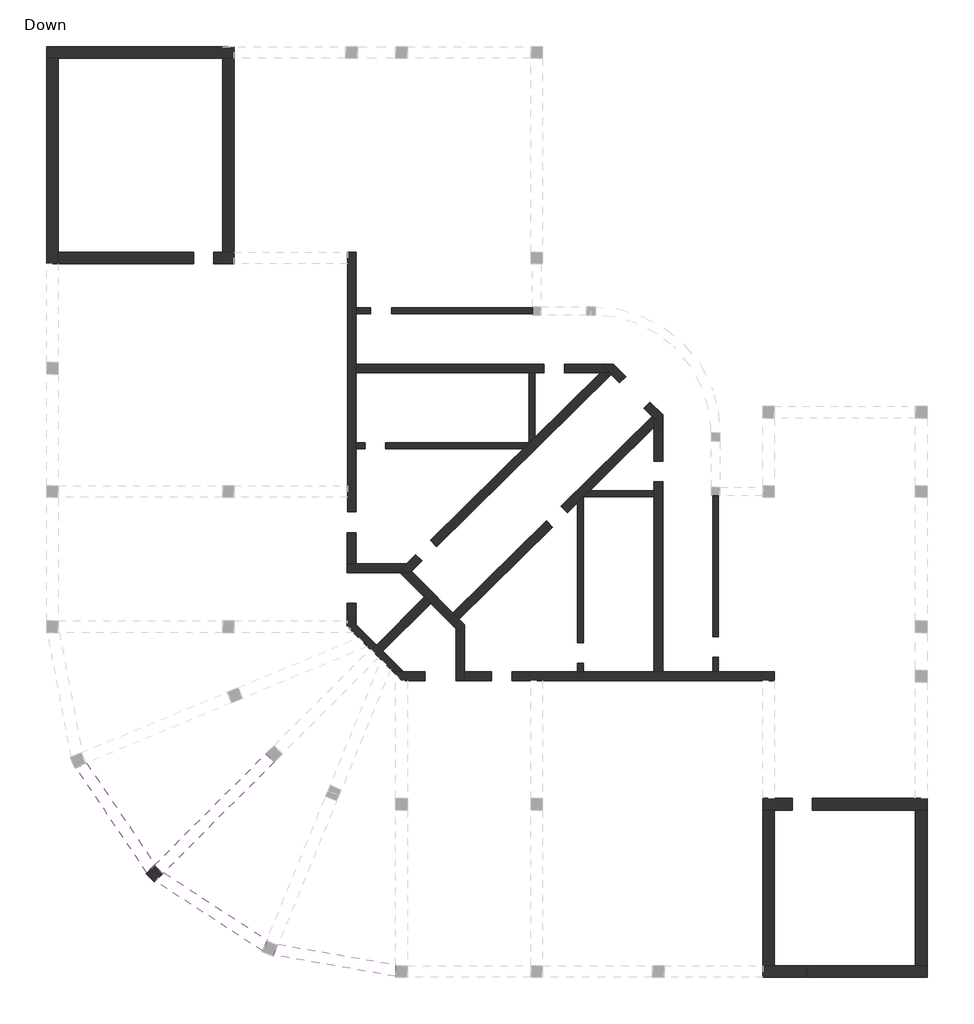
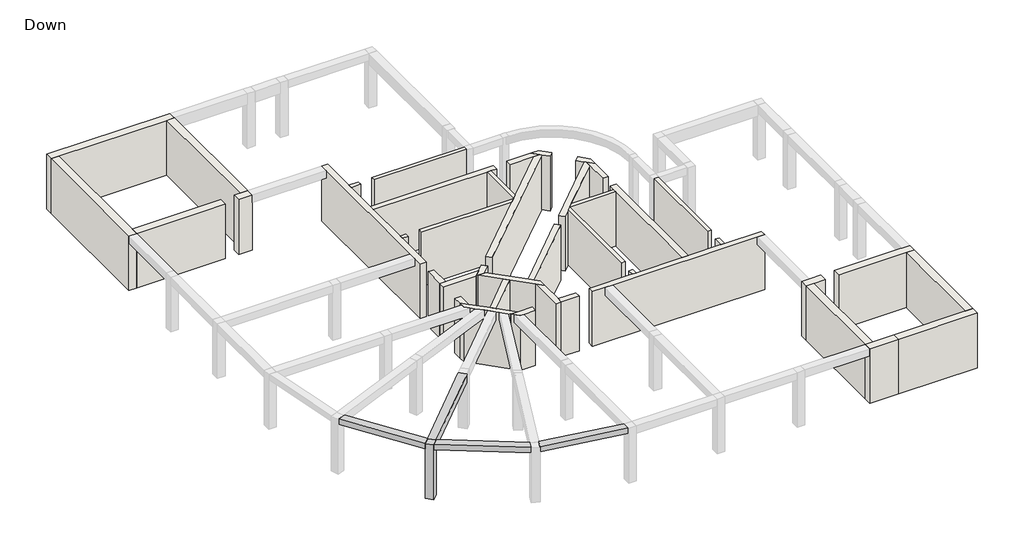
# One storey, part 1 of 2: 42 walls, 4 beams, 1 column.
"""IFC4 building model written with IfcOpenShell, lengths in millimetres."""

from ifc_helpers import new_model, si_unit, origin, origin_with_axes, place, context, project, spatial, polyline, outline, extrude, faceted_brep, element, save

model = new_model("IFC4")

# Units and contexts
model_context = context("Model", 3, world=origin())
ifc_project = project(units=[si_unit("LENGTHUNIT", "METRE", prefix="MILLI")], contexts=[model_context])

# Site, building, storey
site = spatial("IfcSite", under=ifc_project)
building = spatial("IfcBuilding", under=site)
storey = spatial("IfcBuildingStorey", under=building, Name="Down", Elevation=0.0)

# Beams
placement = place(None, origin())
element("IfcBeam", 1, ObjectType="Concrete Rectengular Beam : 39/30", at=placement, inside=storey, context=model_context, shape_type="Brep", body=[
    faceted_brep([(-10715.118829, -3249.9785454, 3000.0), (-10744.371321, -3279.2310368, 3000.0), (-10997.081006, -3531.9407164, 3000.0), (-7342.0637038, -5902.9717923, 3000.0), (-7204.9594265, -5567.8069151, 3000.0), (-7191.7801663, -5535.5889186, 3000.0), (-7191.7801663, -5535.5889186, 2800.0), (-7191.7801663, -5535.5889186, 2700.0), (-10715.118829, -3249.9785454, 2700.0), (-10715.118829, -3249.9785454, 2800.0), (-10997.081006, -3531.9407164, 2700.0), (-7342.0637038, -5902.9717923, 2700.0)], [[[0, 1, 2, 3, 4, 5]], [[0, 5, 6, 7, 8, 9]], [[10, 8, 7, 11]], [[2, 10, 11, 3]], [[10, 2, 1, 0, 9, 8]], [[3, 11, 7, 6, 5, 4]]]),
])
element("IfcBeam", 2, ObjectType="Concrete Rectengular Beam : 39/30", at=placement, inside=storey, context=model_context, shape_type="Brep", body=[
    faceted_brep([(-13331.7826338, 480.4747094, 3000.0), (-13367.6133817, 465.6307069, 3000.0), (-13699.4952625, 328.1383075, 3000.0), (-11282.6282398, -3251.8025252, 3000.0), (-11027.2140258, -2996.3883167, 3000.0), (-11001.7177394, -2970.8920309, 3000.0), (-11001.7177394, -2970.8920309, 2800.0), (-11001.7177394, -2970.8920309, 2700.0), (-13331.7826338, 480.4747094, 2700.0), (-13331.7826338, 480.4747094, 2800.0), (-13699.4952625, 328.1383075, 2700.0), (-11282.6282398, -3251.8025252, 2700.0)], [[[0, 1, 2, 3, 4, 5]], [[0, 5, 6, 7, 8, 9]], [[10, 8, 7, 11]], [[2, 10, 11, 3]], [[10, 2, 1, 0, 9, 8]], [[3, 11, 7, 6, 5, 4]]]),
])
element("IfcBeam", 3, ObjectType="Concrete Rectengular Beam : 39/30", at=placement, inside=storey, context=model_context, shape_type="Brep", body=[
    faceted_brep([(-2813.8658054, -6775.1305116, 3000.0), (-2813.8658054, -6410.076772, 3000.0), (-2813.8658054, -6379.2217224, 3000.0), (-6818.4727302, -5679.49154, 3000.0), (-6834.7373046, -5719.2518901, 3000.0), (-6969.6216332, -6048.9898845, 3000.0), (-2813.8658054, -6775.1305116, 2700.0), (-6969.6216332, -6048.9898845, 2700.0), (-2813.8658054, -6379.2217224, 2700.0), (-6818.4727302, -5679.49154, 2700.0), (-2813.8658054, -6379.2217224, 2800.0), (-6818.4727302, -5679.49154, 2800.0)], [[[0, 1, 2, 3, 4, 5]], [[6, 0, 5, 7]], [[8, 6, 7, 9]], [[3, 2, 10, 8, 9, 11]], [[0, 6, 8, 10, 2, 1]], [[7, 5, 4, 3, 11, 9]]]),
])
element("IfcBeam", 4, ObjectType="Concrete Rectengular Beam : 40/40", at=placement, inside=storey, context=model_context, shape_type="Brep", body=[
    faceted_brep([(-11027.2140255, -2996.388317, 3000.0), (-10744.3713207, -3279.2310371, 3000.0), (-10715.118829, -3249.9785454, 3000.0), (-6954.333921, 510.8063626, 3000.0), (-7237.1766258, 793.6490827, 3000.0), (-11001.7177394, -2970.8920309, 3000.0), (-10744.3713207, -3279.2310371, 2600.0), (-6954.333921, 510.8063626, 2600.0), (-6954.333921, 510.8063626, 2800.0), (-11027.2140255, -2996.388317, 2600.0), (-7237.1766258, 793.6490827, 2600.0), (-7237.1766258, 793.6490827, 2800.0)], [[[0, 1, 2, 3, 4, 5]], [[1, 6, 7, 8, 3, 2]], [[6, 9, 10, 7]], [[9, 0, 5, 4, 11, 10]], [[1, 0, 9, 6]], [[4, 3, 8, 7, 10, 11]]]),
])

# Column
element("IfcColumn", 5, ObjectType="Concrete Rectengular Column : 40/40", at=placement, inside=storey, context=model_context, shape_type="SweptSolid", body=[
    extrude(outline(polyline([(-10744.3713169, -3279.2310409), (-11027.2140369, -3562.0737458), (-11310.0567418, -3279.2310257), (-11027.2140217, -2996.3883208), (-10744.3713169, -3279.2310409)])), origin_with_axes(), (0.0, 0.0, 1.0), 3000.0),
])

# Walls
element("IfcWall", 6, ObjectType="20", at=placement, inside=storey, context=model_context, shape_type="Brep", body=[
    faceted_brep([(-4161.7067397, 15761.3377606, 0.0), (-3665.2660617, 15761.3377606, 0.0), (-3665.2660617, 15761.3377606, 2800.0), (-3665.2660617, 15761.3377606, 3000.0), (-4161.7067397, 15761.3377606, 3000.0), (-4161.7067397, 15761.3377606, 2800.0), (-4161.7067397, 15961.3377606, 0.0), (-4161.7067397, 15961.3377606, 2800.0), (-4161.7067397, 15961.3377606, 3000.0), (-3665.2660617, 15961.3377606, 3000.0), (-3665.2660617, 15961.3377606, 2800.0), (-3665.2660617, 15961.3377606, 0.0)], [[[0, 1, 2, 3, 4, 5]], [[6, 7, 8, 9, 10, 11]], [[1, 0, 6, 11]], [[3, 2, 1, 11, 10, 9]], [[4, 3, 9, 8]], [[0, 5, 4, 8, 7, 6]]]),
])
element("IfcWall", 7, ObjectType="20", at=placement, inside=storey, context=model_context, shape_type="Brep", body=[
    faceted_brep([(-2964.398431, 15761.3377606, 0.0), (1829.020722, 15761.3377606, 0.0), (1829.020722, 15761.3377606, 2800.0), (1829.020722, 15761.3377606, 3000.0), (-2964.398431, 15761.3377606, 3000.0), (-2964.398431, 15761.3377606, 2800.0), (-2964.398431, 15961.3377606, 0.0), (-2964.398431, 15961.3377606, 2800.0), (-2964.398431, 15961.3377606, 3000.0), (1829.020722, 15961.3377606, 3000.0), (1829.020722, 15961.3377606, 2800.0), (1829.020722, 15961.3377606, 0.0)], [[[0, 1, 2, 3, 4, 5]], [[6, 7, 8, 9, 10, 11]], [[1, 0, 6, 11]], [[3, 2, 1, 11, 10, 9]], [[4, 3, 9, 8]], [[0, 5, 4, 8, 7, 6]]]),
])
element("IfcWall", 8, ObjectType="20", at=placement, inside=storey, context=model_context, shape_type="Brep", body=[
    faceted_brep([(8168.0773416, 3579.3391577, 0.0), (8168.0773416, 4078.4432768, 0.0), (8168.0773416, 4078.4432768, 2800.0), (8168.0773416, 4078.4432768, 3000.0), (8168.0773416, 3579.3391577, 3000.0), (8168.0773416, 3579.3391577, 2800.0), (7968.0773416, 3579.3391577, 0.0), (7968.0773416, 3579.3391577, 2800.0), (7968.0773416, 3579.3391577, 3000.0), (7968.0773416, 4078.4432768, 3000.0), (7968.0773416, 4078.4432768, 2800.0), (7968.0773416, 4078.4432768, 0.0)], [[[0, 1, 2, 3, 4, 5]], [[6, 7, 8, 9, 10, 11]], [[1, 0, 6, 11]], [[3, 2, 1, 11, 10, 9]], [[4, 3, 9, 8]], [[0, 5, 4, 8, 7, 6]]]),
])
element("IfcWall", 9, ObjectType="20", at=placement, inside=storey, context=model_context, shape_type="Brep", body=[
    faceted_brep([(8168.0773416, 4779.3109075, 0.0), (8168.0773416, 9562.1590026, 0.0), (8168.0773416, 9562.1590026, 2800.0), (8168.0773416, 9562.1590026, 3000.0), (8168.0773416, 4779.3109075, 3000.0), (8168.0773416, 4779.3109075, 2800.0), (7968.0773416, 4779.3109075, 0.0), (7968.0773416, 4779.3109075, 2800.0), (7968.0773416, 4779.3109075, 3000.0), (7968.0773416, 9562.1590026, 3000.0), (7968.0773416, 9562.1590026, 2800.0), (7968.0773416, 9562.1590026, 0.0)], [[[0, 1, 2, 3, 4, 5]], [[6, 7, 8, 9, 10, 11]], [[1, 0, 6, 11]], [[3, 2, 1, 11, 10, 9]], [[4, 3, 9, 8]], [[0, 5, 4, 8, 7, 6]]]),
])
element("IfcWall", 10, ObjectType="20", at=placement, inside=storey, context=model_context, shape_type="Brep", body=[
    faceted_brep([(3575.2686355, 3579.3391577, 0.0), (3575.2686355, 3876.6777409, 0.0), (3575.2686355, 3876.6777409, 2800.0), (3575.2686355, 3876.6777409, 3000.0), (3575.2686355, 3579.3391577, 3000.0), (3375.2686355, 3579.3391577, 0.0), (3375.2686355, 3579.3391577, 2800.0), (3375.2686355, 3579.3391577, 3000.0), (3375.2686355, 3876.6777409, 3000.0), (3375.2686355, 3876.6777409, 2800.0), (3375.2686355, 3876.6777409, 0.0)], [[[0, 1, 2, 3, 4]], [[5, 6, 7, 8, 9, 10]], [[1, 0, 5, 10]], [[3, 2, 1, 10, 9, 8]], [[4, 3, 8, 7]], [[0, 4, 7, 6, 5]]]),
])
element("IfcWall", 11, ObjectType="20", at=placement, inside=storey, context=model_context, shape_type="Brep", body=[
    faceted_brep([(3575.2686355, 4577.5453716, 0.0), (3575.2686355, 9542.9641204, 0.0), (3575.2686355, 9542.9641204, 3000.0), (3575.2686355, 4577.5453716, 3000.0), (3575.2686355, 4577.5453716, 2800.0), (3375.2686355, 4577.5453716, 0.0), (3375.2686355, 4577.5453716, 2800.0), (3375.2686355, 4577.5453716, 3000.0), (3375.2686355, 9345.8487309, 3000.0), (3375.2686355, 9345.8487309, 2800.0), (3375.2686355, 9345.8487309, 0.0)], [[[0, 1, 2, 3, 4]], [[5, 6, 7, 8, 9, 10]], [[1, 0, 5, 10]], [[3, 2, 8, 7]], [[0, 4, 3, 7, 6, 5]], [[2, 1, 10, 9, 8]]]),
])
element("IfcWall", 12, ObjectType="20", at=placement, inside=storey, context=model_context, shape_type="Brep", body=[
    faceted_brep([(3575.1662411, 9542.8632028, 0.0), (5969.003497, 9542.8632028, 0.0), (5969.003497, 9542.8632028, 3000.0), (3575.1662411, 9542.8632028, 3000.0), (3778.0930653, 9742.8632028, 0.0), (3778.0930653, 9742.8632028, 2800.0), (3778.0930653, 9742.8632028, 3000.0), (5969.003497, 9742.8632028, 3000.0), (5969.003497, 9742.8632028, 2800.0), (5969.003497, 9742.8632028, 0.0)], [[[0, 1, 2, 3]], [[4, 5, 6, 7, 8, 9]], [[1, 0, 4, 9]], [[3, 2, 7, 6]], [[0, 3, 6, 5, 4]], [[2, 1, 9, 8, 7]]]),
])
element("IfcWall", 13, ObjectType="20", at=placement, inside=storey, context=model_context, shape_type="Brep", body=[
    faceted_brep([(-3861.7208648, 11366.7645142, 0.0), (-4161.7067397, 11366.7645142, 0.0), (-4161.7067397, 11366.7645142, 3000.0), (-3861.7208648, 11366.7645142, 3000.0), (-3861.7208648, 11366.7645142, 2800.0), (-3861.7208648, 11166.7645142, 0.0), (-3861.7208648, 11166.7645142, 2800.0), (-3861.7208648, 11166.7645142, 3000.0), (-4161.7067397, 11166.7645142, 3000.0), (-4161.7067397, 11166.7645142, 2800.0), (-4161.7067397, 11166.7645142, 0.0)], [[[0, 1, 2, 3, 4]], [[5, 6, 7, 8, 9, 10]], [[1, 0, 5, 10]], [[3, 2, 8, 7]], [[0, 4, 3, 7, 6, 5]], [[2, 1, 10, 9, 8]]]),
])
element("IfcWall", 14, ObjectType="20", at=placement, inside=storey, context=model_context, shape_type="Brep", body=[
    faceted_brep([(-3166.1629714, 11166.7645142, 0.0), (1521.6521635, 11166.7645142, 0.0), (1521.6521635, 11166.7645142, 2800.0), (1521.6521635, 11166.7645142, 3000.0), (-3166.1629714, 11166.7645142, 3000.0), (-3166.1629714, 11166.7645142, 2800.0), (-3166.1629714, 11366.7645142, 0.0), (-3166.1629714, 11366.7645142, 2800.0), (-3166.1629714, 11366.7645142, 3000.0), (1724.8242608, 11366.7645142, 3000.0), (1724.8242608, 11366.7645142, 0.0)], [[[0, 1, 2, 3, 4, 5]], [[6, 7, 8, 9, 10]], [[1, 0, 6, 10]], [[4, 3, 9, 8]], [[0, 5, 4, 8, 7, 6]], [[3, 2, 1, 10, 9]]]),
])
element("IfcWall", 15, ObjectType="20", at=placement, inside=storey, context=model_context, shape_type="Brep", body=[
    faceted_brep([(1924.8242608, 11563.6419424, 0.0), (1924.8242608, 13749.3760398, 0.0), (1924.8242608, 13749.3760398, 2800.0), (1924.8242608, 13749.3760398, 3000.0), (1924.8242608, 11563.6419424, 3000.0), (1924.8242608, 11563.6419424, 2800.0), (1724.8242608, 11366.7645142, 0.0), (1724.8242608, 11366.7645142, 3000.0), (1724.8242608, 13749.3760398, 3000.0), (1724.8242608, 13749.3760398, 0.0)], [[[0, 1, 2, 3, 4, 5]], [[6, 7, 8, 9]], [[1, 0, 6, 9]], [[4, 3, 8, 7]], [[3, 2, 1, 9, 8]], [[0, 5, 4, 7, 6]]]),
])
element("IfcWall", 16, ObjectType="25", at=placement, inside=storey, context=model_context, shape_type="Brep", body=[
    faceted_brep([(-2555.5586507, 3579.3391577, 0.0), (-3256.6787431, 4280.4592501, 0.0), (-3468.8107774, 4492.5912844, 0.0), (-4167.7621118, 5191.5426188, 0.0), (-4467.7621118, 5491.5426188, 0.0), (-4467.7621118, 5491.5426188, 3000.0), (-4167.7621118, 5191.5426188, 3000.0), (-3468.8107774, 4492.5912844, 3000.0), (-3256.6787431, 4280.4592501, 3000.0), (-2555.5586507, 3579.3391577, 3000.0), (-2555.5586507, 3579.3391577, 2800.0), (-2909.1120413, 3579.3391577, 0.0), (-2909.1120413, 3579.3391577, 3000.0), (-2995.6201329, 3665.8472494, 3000.0), (-3302.3291451, 3972.5562616, 3000.0), (-3397.4447571, 4067.6718736, 3000.0), (-3680.299296, 4350.5264125, 3000.0), (-3771.0702765, 4441.2973929, 3000.0), (-4077.2097101, 4747.4368266, 3000.0), (-4249.2842956, 4919.511412, 3000.0), (-4467.7621118, 5137.9892282, 3000.0), (-4467.7621118, 5137.9892282, 2600.0), (-4467.7621118, 5137.9892282, 0.0), (-4467.7621118, 5319.511412, 3000.0)], [[[0, 1, 2, 3, 4, 5, 6, 7, 8, 9, 10]], [[11, 12, 13, 14, 15, 16, 17, 18, 19, 20, 21, 22]], [[4, 3, 2, 1, 0, 11, 22]], [[9, 8, 7, 6, 5, 23, 20, 19, 18, 17, 16, 15, 14, 13, 12]], [[0, 10, 9, 12, 11]], [[5, 4, 22, 21, 20, 23]]]),
])
element("IfcWall", 17, ObjectType="30", at=placement, inside=storey, context=model_context, shape_type="Brep", body=[
    faceted_brep([(-1817.5239543, 3579.3391577, 0.0), (-2555.5586507, 3579.3391577, 0.0), (-2909.1120413, 3579.3391577, 0.0), (-2909.1120413, 3579.3391577, 3000.0), (-2555.5586507, 3579.3391577, 3000.0), (-1817.5239543, 3579.3391577, 3000.0), (-1817.5239543, 3579.3391577, 2800.0), (-1817.5239543, 3279.3391577, 0.0), (-1817.5239543, 3279.3391577, 2800.0), (-1817.5239543, 3279.3391577, 3000.0), (-2413.8658054, 3279.3391577, 3000.0), (-2609.1120413, 3279.3391577, 3000.0), (-2609.1120413, 3279.3391577, 2600.0), (-2609.1120413, 3279.3391577, 0.0), (-2813.8658054, 3484.0929218, 3000.0)], [[[0, 1, 2, 3, 4, 5, 6]], [[7, 8, 9, 10, 11, 12, 13]], [[2, 1, 0, 7, 13]], [[5, 4, 3, 14, 11, 10, 9]], [[0, 6, 5, 9, 8, 7]], [[3, 2, 13, 12, 11, 14]]]),
])
element("IfcWall", 18, ObjectType="30", at=placement, inside=storey, context=model_context, shape_type="Brep", body=[
    faceted_brep([(-4167.7621118, 5191.5426188, 0.0), (-4167.7621118, 5921.5426188, 0.0), (-4167.7621118, 5921.5426188, 2800.0), (-4167.7621118, 5921.5426188, 3000.0), (-4167.7621118, 5191.5426188, 3000.0), (-4167.7621118, 5191.5426188, 2800.0), (-4467.7621118, 5491.5426188, 0.0), (-4467.7621118, 5491.5426188, 3000.0), (-4467.7621118, 5921.5426188, 3000.0), (-4467.7621118, 5921.5426188, 2800.0), (-4467.7621118, 5921.5426188, 0.0)], [[[0, 1, 2, 3, 4, 5]], [[6, 7, 8, 9, 10]], [[1, 0, 6, 10]], [[3, 2, 1, 10, 9, 8]], [[4, 3, 8, 7]], [[0, 5, 4, 7, 6]]]),
])
element("IfcWall", 19, ObjectType="30", at=placement, inside=storey, context=model_context, shape_type="Brep", body=[
    faceted_brep([(-3256.6787431, 4280.4592501, 0.0), (-1621.3195657, 5915.8184274, 0.0), (-1621.3195657, 5915.8184274, 2800.0), (-1621.3195657, 5915.8184274, 3000.0), (-3256.6787431, 4280.4592501, 3000.0), (-3256.6787431, 4280.4592501, 2800.0), (-3468.8107774, 4492.5912844, 0.0), (-3468.8107774, 4492.5912844, 2800.0), (-3468.8107774, 4492.5912844, 3000.0), (-1833.4516001, 6127.9504618, 3000.0), (-1833.4516001, 6127.9504618, 2800.0), (-1833.4516001, 6127.9504618, 0.0)], [[[0, 1, 2, 3, 4, 5]], [[6, 7, 8, 9, 10, 11]], [[1, 0, 6, 11]], [[4, 3, 9, 8]], [[0, 5, 4, 8, 7, 6]], [[3, 2, 1, 11, 10, 9]]]),
])
element("IfcWall", 20, ObjectType="30", at=placement, inside=storey, context=model_context, shape_type="Brep", body=[
    faceted_brep([(-2664.82245, 6959.3213117, 0.0), (-1833.4516001, 6127.9504618, 0.0), (-1621.3195657, 5915.8184274, 0.0), (-769.9852407, 5064.4841024, 0.0), (-469.9852407, 4764.4841024, 0.0), (-469.9852407, 4764.4841024, 3000.0), (-769.9852407, 5064.4841024, 3000.0), (-1621.3195657, 5915.8184274, 3000.0), (-1833.4516001, 6127.9504618, 3000.0), (-2664.82245, 6959.3213117, 3000.0), (-2664.82245, 6959.3213117, 2800.0), (-469.9852407, 5188.7481711, 0.0), (-654.972774, 5373.7357044, 0.0), (-867.1104047, 5585.8733352, 0.0), (-2282.3881282, 7001.1510587, 0.0), (-2282.3881282, 7001.1510587, 3000.0), (-867.1104047, 5585.8733352, 3000.0), (-654.972774, 5373.7357044, 3000.0), (-469.9852407, 5188.7481711, 3000.0), (-469.9852407, 5188.7481711, 2800.0), (-2324.8813154, 6959.3213117, 0.0), (-2324.8813154, 6959.3213117, 3000.0)], [[[0, 1, 2, 3, 4, 5, 6, 7, 8, 9, 10]], [[11, 12, 13, 14, 15, 16, 17, 18, 19]], [[4, 3, 2, 1, 0, 20, 14, 13, 12, 11]], [[9, 8, 7, 6, 5, 18, 17, 16, 15, 21]], [[5, 4, 11, 19, 18]], [[0, 10, 9, 21, 20]], [[15, 14, 20, 21]]]),
])
element("IfcWall", 21, ObjectType="30", at=placement, inside=storey, context=model_context, shape_type="Brep", body=[
    faceted_brep([(-769.9852407, 5064.4841024, 0.0), (-769.9852407, 3279.3391577, 0.0), (-769.9852407, 3279.3391577, 2800.0), (-769.9852407, 3279.3391577, 3000.0), (-769.9852407, 5064.4841024, 3000.0), (-769.9852407, 5064.4841024, 2800.0), (-469.9852407, 4764.4841024, 0.0), (-469.9852407, 4764.4841024, 3000.0), (-469.9852407, 3579.3391577, 3000.0), (-469.9852407, 3279.3391577, 3000.0), (-469.9852407, 3279.3391577, 0.0), (-469.9852407, 3579.3391577, 0.0)], [[[0, 1, 2, 3, 4, 5]], [[6, 7, 8, 9, 10, 11]], [[1, 0, 6, 11, 10]], [[4, 3, 9, 8, 7]], [[0, 5, 4, 7, 6]], [[3, 2, 1, 10, 9]]]),
])
element("IfcWall", 22, ObjectType="30", at=placement, inside=storey, context=model_context, shape_type="Brep", body=[
    faceted_brep([(-469.9852407, 3279.3391577, 0.0), (450.0147593, 3279.3391577, 0.0), (450.0147593, 3279.3391577, 2800.0), (450.0147593, 3279.3391577, 3000.0), (-469.9852407, 3279.3391577, 3000.0), (-469.9852407, 3579.3391577, 0.0), (-469.9852407, 3579.3391577, 2800.0), (-469.9852407, 3579.3391577, 3000.0), (450.0147593, 3579.3391577, 3000.0), (450.0147593, 3579.3391577, 2800.0), (450.0147593, 3579.3391577, 0.0)], [[[0, 1, 2, 3, 4]], [[5, 6, 7, 8, 9, 10]], [[1, 0, 5, 10]], [[3, 2, 1, 10, 9, 8]], [[4, 3, 8, 7]], [[0, 4, 7, 6, 5]]]),
])
element("IfcWall", 23, ObjectType="30", at=placement, inside=storey, context=model_context, shape_type="Brep", body=[
    faceted_brep([(1134.6168888, 3279.3391577, 0.0), (10069.6339123, 3279.3391577, 0.0), (10069.6339123, 3279.3391577, 2600.0), (10069.6339123, 3279.3391577, 3000.0), (9669.6339123, 3279.3391577, 3000.0), (2179.020722, 3279.3391577, 3000.0), (1779.020722, 3279.3391577, 3000.0), (1134.6168888, 3279.3391577, 3000.0), (1134.6168888, 3279.3391577, 2800.0), (1134.6168888, 3579.3391577, 0.0), (1134.6168888, 3579.3391577, 2800.0), (1134.6168888, 3579.3391577, 3000.0), (3375.2686355, 3579.3391577, 3000.0), (3575.2686355, 3579.3391577, 3000.0), (5969.003497, 3579.3391577, 3000.0), (6269.003497, 3579.3391577, 3000.0), (7968.0773416, 3579.3391577, 3000.0), (8168.0773416, 3579.3391577, 3000.0), (10069.6339123, 3579.3391577, 3000.0), (10069.6339123, 3579.3391577, 2800.0), (10069.6339123, 3579.3391577, 0.0), (8168.0773416, 3579.3391577, 0.0), (7968.0773416, 3579.3391577, 0.0), (6269.003497, 3579.3391577, 0.0), (5969.003497, 3579.3391577, 0.0), (3575.2686355, 3579.3391577, 0.0), (3375.2686355, 3579.3391577, 0.0)], [[[0, 1, 2, 3, 4, 5, 6, 7, 8]], [[9, 10, 11, 12, 13, 14, 15, 16, 17, 18, 19, 20, 21, 22, 23, 24, 25, 26]], [[1, 0, 9, 26, 25, 24, 23, 22, 21, 20]], [[3, 2, 1, 20, 19, 18]], [[7, 6, 5, 4, 3, 18, 17, 16, 15, 14, 13, 12, 11]], [[0, 8, 7, 11, 10, 9]]]),
])
element("IfcWall", 24, ObjectType="30", at=placement, inside=storey, context=model_context, shape_type="SweptSolid", body=[
    extrude(outline(polyline([(2521.8013373, 8504.6910362), (-654.972774, 5373.7357044), (-867.1104047, 5585.8733352), (2311.2157666, 8718.3583416), (2521.8013373, 8504.6910362)])), origin_with_axes(), (0.0, 0.0, 1.0), 3000.0),
])
element("IfcWall", 25, ObjectType="30", at=placement, inside=storey, context=model_context, shape_type="Brep", body=[
    faceted_brep([(3019.4754557, 8995.1871747, 0.0), (3375.2686355, 9345.8487309, 0.0), (3575.2686355, 9542.9641204, 0.0), (3778.0930653, 9742.8632028, 0.0), (5969.003497, 11902.1740186, 0.0), (5969.003497, 11902.1740186, 2800.0), (5969.003497, 11902.1740186, 3000.0), (3778.0930653, 9742.8632028, 3000.0), (3575.2686355, 9542.9641204, 3000.0), (3375.2686355, 9345.8487309, 3000.0), (3019.4754557, 8995.1871747, 3000.0), (3019.4754557, 8995.1871747, 2800.0), (2808.889885, 9208.8544801, 0.0), (2808.889885, 9208.8544801, 3000.0), (5906.8587116, 12262.1411401, 3000.0), (5906.8587116, 12262.1411401, 0.0), (5969.003497, 12199.9963547, 0.0), (5969.003497, 12199.9963547, 3000.0), (2897.8940684, 9118.5477987, 3000.0)], [[[0, 1, 2, 3, 4, 5, 6, 7, 8, 9, 10, 11]], [[12, 13, 14, 15]], [[4, 3, 2, 1, 0, 12, 15, 16]], [[10, 9, 8, 7, 6, 17, 14, 13, 18]], [[0, 11, 10, 18, 13, 12]], [[6, 5, 4, 16, 17]], [[16, 15, 14, 17]]]),
])
element("IfcWall", 26, ObjectType="30", at=placement, inside=storey, context=model_context, shape_type="Brep", body=[
    faceted_brep([(-2447.7649909, 7259.3213117, 0.0), (-4167.7621118, 7259.3213117, 0.0), (-4467.7621118, 7259.3213117, 0.0), (-4467.7621118, 7259.3213117, 3000.0), (-4167.7621118, 7259.3213117, 3000.0), (-2447.7649909, 7259.3213117, 3000.0), (-2447.7649909, 7259.3213117, 2800.0), (-2752.523137, 6959.3213117, 0.0), (-2752.523137, 6959.3213117, 3000.0), (-4467.7621118, 6959.3213117, 3000.0), (-4467.7621118, 6959.3213117, 2800.0), (-4467.7621118, 6959.3213117, 0.0)], [[[0, 1, 2, 3, 4, 5, 6]], [[7, 8, 9, 10, 11]], [[2, 1, 0, 7, 11]], [[5, 4, 3, 9, 8]], [[3, 2, 11, 10, 9]], [[0, 6, 5, 8, 7]]]),
])
element("IfcWall", 27, ObjectType="30", at=placement, inside=storey, context=model_context, shape_type="Brep", body=[
    faceted_brep([(-4167.7621118, 7259.3213117, 0.0), (-4167.7621118, 8319.3213117, 0.0), (-4167.7621118, 8319.3213117, 2800.0), (-4167.7621118, 8319.3213117, 3000.0), (-4167.7621118, 7259.3213117, 3000.0), (-4167.7621118, 7259.3213117, 2800.0), (-4467.7621118, 7259.3213117, 0.0), (-4467.7621118, 7259.3213117, 3000.0), (-4467.7621118, 8319.3213117, 3000.0), (-4467.7621118, 8319.3213117, 2800.0), (-4467.7621118, 8319.3213117, 0.0), (-4317.7621118, 8319.3213117, 3000.0)], [[[0, 1, 2, 3, 4, 5]], [[6, 7, 8, 9, 10]], [[1, 0, 6, 10]], [[3, 2, 1, 10, 9, 8, 11]], [[4, 3, 11, 8, 7]], [[0, 5, 4, 7, 6]]]),
])
element("IfcWall", 28, ObjectType="30", at=placement, inside=storey, context=model_context, shape_type="Brep", body=[
    faceted_brep([(-4161.7067397, 9032.3032318, 0.0), (-4161.7067397, 11166.7645142, 0.0), (-4161.7067397, 11366.7645142, 0.0), (-4161.7067397, 13749.3760398, 0.0), (-4161.7067397, 14049.3760398, 0.0), (-4161.7067397, 15761.3377606, 0.0), (-4161.7067397, 15961.3377606, 0.0), (-4161.7067397, 17856.8664083, 0.0), (-4161.7067397, 17856.8664083, 2800.0), (-4161.7067397, 17856.8664083, 3000.0), (-4161.7067397, 15961.3377606, 3000.0), (-4161.7067397, 15761.3377606, 3000.0), (-4161.7067397, 14049.3760398, 3000.0), (-4161.7067397, 13749.3760398, 3000.0), (-4161.7067397, 11366.7645142, 3000.0), (-4161.7067397, 11166.7645142, 3000.0), (-4161.7067397, 9032.3032318, 3000.0), (-4161.7067397, 9032.3032318, 2800.0), (-4461.7067397, 9032.3032318, 0.0), (-4461.7067397, 9032.3032318, 2800.0), (-4461.7067397, 9032.3032318, 3000.0), (-4461.7067397, 9512.1590026, 3000.0), (-4461.7067397, 9912.1590026, 3000.0), (-4461.7067397, 17456.8664083, 3000.0), (-4461.7067397, 17856.8664083, 3000.0), (-4461.7067397, 17856.8664083, 2600.0), (-4461.7067397, 17856.8664083, 0.0), (-4317.7621118, 9032.3032318, 3000.0)], [[[0, 1, 2, 3, 4, 5, 6, 7, 8, 9, 10, 11, 12, 13, 14, 15, 16, 17]], [[18, 19, 20, 21, 22, 23, 24, 25, 26]], [[7, 6, 5, 4, 3, 2, 1, 0, 18, 26]], [[9, 8, 7, 26, 25, 24]], [[16, 15, 14, 13, 12, 11, 10, 9, 24, 23, 22, 21, 20, 27]], [[0, 17, 16, 27, 20, 19, 18]]]),
])
element("IfcWall", 29, ObjectType="30", at=placement, inside=storey, context=model_context, shape_type="Brep", body=[
    faceted_brep([(5969.003497, 10041.1289202, 0.0), (5969.003497, 9742.8632028, 0.0), (5969.003497, 9542.8632028, 0.0), (5969.003497, 3579.3391577, 0.0), (5969.003497, 3579.3391577, 3000.0), (5969.003497, 9542.8632028, 3000.0), (5969.003497, 9742.8632028, 3000.0), (5969.003497, 10041.1289202, 3000.0), (5969.003497, 10041.1289202, 2800.0), (6269.003497, 10041.1289202, 0.0), (6269.003497, 10041.1289202, 2800.0), (6269.003497, 10041.1289202, 3000.0), (6269.003497, 3579.3391577, 3000.0), (6269.003497, 3579.3391577, 2800.0), (6269.003497, 3579.3391577, 0.0)], [[[0, 1, 2, 3, 4, 5, 6, 7, 8]], [[9, 10, 11, 12, 13, 14]], [[3, 2, 1, 0, 9, 14]], [[7, 6, 5, 4, 12, 11]], [[0, 8, 7, 11, 10, 9]], [[4, 3, 14, 13, 12]]]),
])
element("IfcWall", 30, ObjectType="30", at=placement, inside=storey, context=model_context, shape_type="Brep", body=[
    faceted_brep([(6269.003497, 10741.9965509, 0.0), (6269.003497, 11899.9963547, 0.0), (6269.003497, 11899.9963547, 3000.0), (6269.003497, 10741.9965509, 3000.0), (6269.003497, 10741.9965509, 2800.0), (5969.003497, 10741.9965509, 0.0), (5969.003497, 10741.9965509, 2800.0), (5969.003497, 10741.9965509, 3000.0), (5969.003497, 11902.1740186, 3000.0), (5969.003497, 12199.9963547, 3000.0), (5969.003497, 12199.9963547, 0.0), (5969.003497, 11902.1740186, 0.0)], [[[0, 1, 2, 3, 4]], [[5, 6, 7, 8, 9, 10, 11]], [[1, 0, 5, 11, 10]], [[3, 2, 9, 8, 7]], [[0, 4, 3, 7, 6, 5]], [[2, 1, 10, 9]]]),
])
element("IfcWall", 31, ObjectType="30", at=placement, inside=storey, context=model_context, shape_type="Brep", body=[
    faceted_brep([(6269.003497, 12324.2604234, 0.0), (5836.2714262, 12756.9924943, 0.0), (5836.2714262, 12756.9924943, 3000.0), (6269.003497, 12324.2604234, 3000.0), (6269.003497, 12324.2604234, 2800.0), (5624.1393918, 12544.8604599, 3000.0), (5624.1393918, 12544.8604599, 0.0), (5906.8587116, 12262.1411401, 0.0), (5969.003497, 12199.9963547, 0.0), (6269.003497, 11899.9963547, 0.0), (6269.003497, 11899.9963547, 3000.0), (5969.003497, 12199.9963547, 3000.0), (5906.8587116, 12262.1411401, 3000.0)], [[[0, 1, 2, 3, 4]], [[5, 6, 7, 8, 9, 10, 11, 12]], [[1, 0, 9, 8, 7, 6]], [[2, 1, 6, 5]], [[3, 2, 5, 12, 11, 10]], [[0, 4, 3, 10, 9]]]),
])
element("IfcWall", 32, ObjectType="30", at=placement, inside=storey, context=model_context, shape_type="Brep", body=[
    faceted_brep([(5010.62779, 13625.111971, 0.0), (4586.3637213, 14049.3760398, 0.0), (4586.3637213, 14049.3760398, 2800.0), (4586.3637213, 14049.3760398, 3000.0), (5010.62779, 13625.111971, 3000.0), (5010.62779, 13625.111971, 2800.0), (4798.4957556, 13412.9799367, 0.0), (4798.4957556, 13412.9799367, 3000.0), (4517.0475694, 13694.4281229, 3000.0), (4462.0996526, 13749.3760398, 3000.0), (4162.0996526, 14049.3760398, 3000.0), (4162.0996526, 14049.3760398, 0.0), (4462.0996526, 13749.3760398, 0.0), (4517.0475694, 13694.4281229, 0.0), (4989.3898697, 13603.8740507, 3000.0)], [[[0, 1, 2, 3, 4, 5]], [[6, 7, 8, 9, 10, 11, 12, 13]], [[1, 0, 6, 13, 12, 11]], [[4, 3, 10, 9, 8, 7, 14]], [[0, 5, 4, 14, 7, 6]], [[3, 2, 1, 11, 10]]]),
])
element("IfcWall", 33, ObjectType="30", at=placement, inside=storey, context=model_context, shape_type="Brep", body=[
    faceted_brep([(4162.0996526, 14049.3760398, 0.0), (2926.3637213, 14049.3760398, 0.0), (2926.3637213, 14049.3760398, 2800.0), (2926.3637213, 14049.3760398, 3000.0), (4162.0996526, 14049.3760398, 3000.0), (4462.0996526, 13749.3760398, 0.0), (4462.0996526, 13749.3760398, 3000.0), (4145.2251653, 13749.3760398, 3000.0), (2926.3637213, 13749.3760398, 3000.0), (2926.3637213, 13749.3760398, 2800.0), (2926.3637213, 13749.3760398, 0.0), (4145.2251653, 13749.3760398, 0.0)], [[[0, 1, 2, 3, 4]], [[5, 6, 7, 8, 9, 10, 11]], [[1, 0, 5, 11, 10]], [[3, 2, 1, 10, 9, 8]], [[4, 3, 8, 7, 6]], [[0, 4, 6, 5]]]),
])
element("IfcWall", 34, ObjectType="30", at=placement, inside=storey, context=model_context, shape_type="Brep", body=[
    faceted_brep([(2223.0854171, 14049.3760398, 0.0), (-4161.7067397, 14049.3760398, 0.0), (-4161.7067397, 14049.3760398, 2800.0), (-4161.7067397, 14049.3760398, 3000.0), (2223.0854171, 14049.3760398, 3000.0), (2223.0854171, 14049.3760398, 2800.0), (2223.0854171, 13749.3760398, 0.0), (2223.0854171, 13749.3760398, 2800.0), (2223.0854171, 13749.3760398, 3000.0), (1924.8242608, 13749.3760398, 3000.0), (1724.8242608, 13749.3760398, 3000.0), (-4161.7067397, 13749.3760398, 3000.0), (-4161.7067397, 13749.3760398, 0.0), (1724.8242608, 13749.3760398, 0.0), (1924.8242608, 13749.3760398, 0.0)], [[[0, 1, 2, 3, 4, 5]], [[6, 7, 8, 9, 10, 11, 12, 13, 14]], [[1, 0, 6, 14, 13, 12]], [[4, 3, 11, 10, 9, 8]], [[0, 5, 4, 8, 7, 6]], [[3, 2, 1, 12, 11]]]),
])
element("IfcWall", 35, ObjectType="30", at=placement, inside=storey, context=model_context, shape_type="Brep", body=[
    faceted_brep([(4145.2251653, 13749.3760398, 0.0), (1924.8242608, 11563.6419424, 0.0), (1724.8242608, 11366.7645142, 0.0), (1521.6521635, 11166.7645142, 0.0), (-1638.9943721, 8055.4647086, 0.0), (-1638.9943721, 8055.4647086, 2800.0), (-1638.9943721, 8055.4647086, 3000.0), (1521.6521635, 11166.7645142, 3000.0), (1724.8242608, 11366.7645142, 3000.0), (1924.8242608, 11563.6419424, 3000.0), (4145.2251653, 13749.3760398, 3000.0), (4145.2251653, 13749.3760398, 2800.0), (-1428.5378745, 7841.6702684, 0.0), (4517.0475694, 13694.4281229, 0.0), (4517.0475694, 13694.4281229, 3000.0), (-1428.5378745, 7841.6702684, 3000.0), (-1428.5378745, 7841.6702684, 2800.0), (4462.0996526, 13749.3760398, 0.0), (4462.0996526, 13749.3760398, 3000.0)], [[[0, 1, 2, 3, 4, 5, 6, 7, 8, 9, 10, 11]], [[12, 13, 14, 15, 16]], [[4, 3, 2, 1, 0, 17, 13, 12]], [[6, 5, 4, 12, 16, 15]], [[10, 9, 8, 7, 6, 15, 14, 18]], [[0, 11, 10, 18, 17]], [[14, 13, 17, 18]]]),
])
element("IfcWall", 36, ObjectType="30", at=placement, inside=storey, context=model_context, shape_type="Brep", body=[
    faceted_brep([(-2134.0535546, 7568.1348155, 0.0), (-2447.7649909, 7259.3213117, 0.0), (-2752.523137, 6959.3213117, 0.0), (-2752.523137, 6959.3213117, 3000.0), (-2447.7649909, 7259.3213117, 3000.0), (-2134.0535546, 7568.1348155, 3000.0), (-2134.0535546, 7568.1348155, 2800.0), (-1923.597057, 7354.3403753, 0.0), (-1923.597057, 7354.3403753, 2800.0), (-1923.597057, 7354.3403753, 3000.0), (-2282.3881282, 7001.1510587, 3000.0), (-2324.8813154, 6959.3213117, 3000.0), (-2324.8813154, 6959.3213117, 0.0), (-2282.3881282, 7001.1510587, 0.0), (-2664.82245, 6959.3213117, 0.0), (-2664.82245, 6959.3213117, 3000.0)], [[[0, 1, 2, 3, 4, 5, 6]], [[7, 8, 9, 10, 11, 12, 13]], [[2, 1, 0, 7, 13, 12, 14]], [[5, 4, 3, 15, 11, 10, 9]], [[0, 6, 5, 9, 8, 7]], [[3, 2, 14, 12, 11, 15]]]),
])
element("IfcWall", 37, ObjectType="40", at=placement, inside=storey, context=model_context, shape_type="Brep", body=[
    faceted_brep([(-8305.861308, 24844.3058567, 0.0), (-14696.6369988, 24844.3058567, 0.0), (-14696.6369988, 24844.3058567, 3000.0), (-8705.861308, 24844.3058567, 3000.0), (-8305.861308, 24844.3058567, 3000.0), (-8305.861308, 24844.3058567, 2400.0), (-8305.861308, 24444.3058567, 0.0), (-8305.861308, 24444.3058567, 3000.0), (-8705.861308, 24444.3058567, 3000.0), (-14296.6369988, 24444.3058567, 3000.0), (-14696.6369988, 24444.3058567, 3000.0), (-14696.6369988, 24444.3058567, 0.0), (-14296.6369988, 24444.3058567, 0.0), (-8705.861308, 24444.3058567, 0.0), (-8305.861308, 24445.393344, 3000.0)], [[[0, 1, 2, 3, 4, 5]], [[6, 7, 8, 9, 10, 11, 12, 13]], [[1, 0, 6, 13, 12, 11]], [[4, 3, 2, 10, 9, 8, 7, 14]], [[0, 5, 4, 14, 7, 6]], [[2, 1, 11, 10]]]),
])
element("IfcWall", 38, ObjectType="40", at=placement, inside=storey, context=model_context, shape_type="Brep", body=[
    faceted_brep([(-14696.6369988, 24444.3058567, 0.0), (-14696.6369988, 17456.8664083, 0.0), (-14696.6369988, 17456.8664083, 2600.0), (-14696.6369988, 17456.8664083, 3000.0), (-14696.6369988, 24444.3058567, 3000.0), (-14296.6369988, 24444.3058567, 0.0), (-14296.6369988, 24444.3058567, 2800.0), (-14296.6369988, 24444.3058567, 3000.0), (-14296.6369988, 17856.8664083, 3000.0), (-14296.6369988, 17456.8664083, 3000.0), (-14296.6369988, 17456.8664083, 2600.0), (-14296.6369988, 17456.8664083, 0.0), (-14296.6369988, 17856.8664083, 0.0)], [[[0, 1, 2, 3, 4]], [[5, 6, 7, 8, 9, 10, 11, 12]], [[1, 0, 5, 12, 11]], [[4, 3, 9, 8, 7]], [[0, 4, 7, 6, 5]], [[3, 2, 1, 11, 10, 9]]]),
])
element("IfcWall", 39, ObjectType="40", at=placement, inside=storey, context=model_context, shape_type="Brep", body=[
    faceted_brep([(-14296.6369988, 17456.8664083, 0.0), (-9693.3146493, 17456.8664083, 0.0), (-9693.3146493, 17456.8664083, 2800.0), (-9693.3146493, 17456.8664083, 3000.0), (-14296.6369988, 17456.8664083, 3000.0), (-14296.6369988, 17456.8664083, 2800.0), (-14296.6369988, 17856.8664083, 0.0), (-14296.6369988, 17856.8664083, 2800.0), (-14296.6369988, 17856.8664083, 3000.0), (-9693.3146493, 17856.8664083, 3000.0), (-9693.3146493, 17856.8664083, 2800.0), (-9693.3146493, 17856.8664083, 0.0)], [[[0, 1, 2, 3, 4, 5]], [[6, 7, 8, 9, 10, 11]], [[1, 0, 6, 11]], [[3, 2, 1, 11, 10, 9]], [[4, 3, 9, 8]], [[0, 5, 4, 8, 7, 6]]]),
])
element("IfcWall", 40, ObjectType="40", at=placement, inside=storey, context=model_context, shape_type="Brep", body=[
    faceted_brep([(-9006.7279431, 17456.8664083, 0.0), (-8305.861308, 17456.8664083, 0.0), (-8305.861308, 17456.8664083, 2600.0), (-8305.861308, 17456.8664083, 3000.0), (-9006.7279431, 17456.8664083, 3000.0), (-9006.7279431, 17456.8664083, 2800.0), (-9006.7279431, 17856.8664083, 0.0), (-9006.7279431, 17856.8664083, 2800.0), (-9006.7279431, 17856.8664083, 3000.0), (-8705.861308, 17856.8664083, 3000.0), (-8305.861308, 17856.8664083, 3000.0), (-8305.861308, 17856.8664083, 2600.0), (-8305.861308, 17856.8664083, 0.0), (-8705.861308, 17856.8664083, 0.0)], [[[0, 1, 2, 3, 4, 5]], [[6, 7, 8, 9, 10, 11, 12, 13]], [[1, 0, 6, 13, 12]], [[4, 3, 10, 9, 8]], [[0, 5, 4, 8, 7, 6]], [[3, 2, 1, 12, 11, 10]]]),
])
element("IfcWall", 41, ObjectType="40", at=placement, inside=storey, context=model_context, shape_type="Brep", body=[
    faceted_brep([(-8305.861308, 17856.8664083, 0.0), (-8305.861308, 24444.3058567, 0.0), (-8305.861308, 24444.3058567, 3000.0), (-8305.861308, 17856.8664083, 3000.0), (-8305.861308, 17856.8664083, 2800.0), (-8705.861308, 17856.8664083, 0.0), (-8705.861308, 17856.8664083, 2800.0), (-8705.861308, 17856.8664083, 3000.0), (-8705.861308, 24444.3058567, 3000.0), (-8705.861308, 24444.3058567, 2800.0), (-8705.861308, 24444.3058567, 0.0)], [[[0, 1, 2, 3, 4]], [[5, 6, 7, 8, 9, 10]], [[1, 0, 5, 10]], [[3, 2, 8, 7]], [[0, 4, 3, 7, 6, 5]], [[2, 1, 10, 9, 8]]]),
])
element("IfcWall", 42, ObjectType="40", at=placement, inside=storey, context=model_context, shape_type="Brep", body=[
    faceted_brep([(9669.6339123, -6810.076772, 0.0), (11162.4147884, -6810.076772, 0.0), (11162.4147884, -6810.076772, 3000.0), (9669.6339123, -6810.076772, 3000.0), (9669.6339123, -6810.076772, 2600.0), (9669.6339123, -6410.076772, 0.0), (9669.6339123, -6410.076772, 2600.0), (9669.6339123, -6410.076772, 3000.0), (10069.6339123, -6410.076772, 3000.0), (11162.4147884, -6410.076772, 3000.0), (11162.4147884, -6410.076772, 0.0), (10069.6339123, -6410.076772, 0.0)], [[[0, 1, 2, 3, 4]], [[5, 6, 7, 8, 9, 10, 11]], [[1, 0, 5, 11, 10]], [[2, 1, 10, 9]], [[3, 2, 9, 8, 7]], [[0, 4, 3, 7, 6, 5]]]),
])
element("IfcWall", 43, ObjectType="40", at=placement, inside=storey, context=model_context, shape_type="Brep", body=[
    faceted_brep([(11162.4147884, -6810.076772, 0.0), (15262.6652109, -6810.076772, 0.0), (15262.6652109, -6810.076772, 3000.0), (11162.4147884, -6810.076772, 3000.0), (11162.4147884, -6410.076772, 0.0), (11162.4147884, -6410.076772, 3000.0), (14862.6652109, -6410.076772, 3000.0), (15262.6652109, -6410.076772, 3000.0), (15262.6652109, -6410.076772, 0.0), (14862.6652109, -6410.076772, 0.0)], [[[0, 1, 2, 3]], [[4, 5, 6, 7, 8, 9]], [[1, 0, 4, 9, 8]], [[3, 2, 7, 6, 5]], [[0, 3, 5, 4]], [[2, 1, 8, 7]]]),
])
element("IfcWall", 44, ObjectType="40", at=placement, inside=storey, context=model_context, shape_type="Brep", body=[
    faceted_brep([(15262.6652109, -6410.076772, 0.0), (15262.6652109, -1116.1309652, 0.0), (15262.6652109, -1116.1309652, 3000.0), (15262.6652109, -6410.076772, 3000.0), (14862.6652109, -6410.076772, 0.0), (14862.6652109, -6410.076772, 2800.0), (14862.6652109, -6410.076772, 3000.0), (14862.6652109, -1116.1309652, 3000.0), (14862.6652109, -1116.1309652, 2800.0), (14862.6652109, -1116.1309652, 0.0)], [[[0, 1, 2, 3]], [[4, 5, 6, 7, 8, 9]], [[1, 0, 4, 9]], [[3, 2, 7, 6]], [[0, 3, 6, 5, 4]], [[2, 1, 9, 8, 7]]]),
])
element("IfcWall", 45, ObjectType="40", at=placement, inside=storey, context=model_context, shape_type="Brep", body=[
    faceted_brep([(15262.6652109, -716.1309652, 0.0), (11362.6652109, -716.1309652, 0.0), (11362.6652109, -716.1309652, 2800.0), (11362.6652109, -716.1309652, 3000.0), (14862.3806142, -716.1309652, 3000.0), (15262.3806142, -716.1309652, 3000.0), (15262.6652109, -716.1309652, 3000.0), (15262.6652109, -1116.1309652, 0.0), (15262.6652109, -1116.1309652, 3000.0), (14862.6652109, -1116.1309652, 3000.0), (11362.6652109, -1116.1309652, 3000.0), (11362.6652109, -1116.1309652, 2800.0), (11362.6652109, -1116.1309652, 0.0), (14862.6652109, -1116.1309652, 0.0)], [[[0, 1, 2, 3, 4, 5, 6]], [[7, 8, 9, 10, 11, 12, 13]], [[1, 0, 7, 13, 12]], [[3, 2, 1, 12, 11, 10]], [[6, 5, 4, 3, 10, 9, 8]], [[0, 6, 8, 7]]]),
])
element("IfcWall", 46, ObjectType="40", at=placement, inside=storey, context=model_context, shape_type="Brep", body=[
    faceted_brep([(10670.3228524, -716.1309652, 0.0), (9669.6339123, -716.1309652, 0.0), (9669.6339123, -716.1309652, 2600.0), (9669.6339123, -716.1309652, 3000.0), (10069.6339123, -716.1309652, 3000.0), (10670.3228524, -716.1309652, 3000.0), (10670.3228524, -716.1309652, 2800.0), (10670.3228524, -1116.1309652, 0.0), (10670.3228524, -1116.1309652, 2800.0), (10670.3228524, -1116.1309652, 3000.0), (10069.6339123, -1116.1309652, 3000.0), (9669.6339123, -1116.1309652, 3000.0), (9669.6339123, -1116.1309652, 0.0), (10069.6339123, -1116.1309652, 0.0)], [[[0, 1, 2, 3, 4, 5, 6]], [[7, 8, 9, 10, 11, 12, 13]], [[1, 0, 7, 13, 12]], [[5, 4, 3, 11, 10, 9]], [[0, 6, 5, 9, 8, 7]], [[3, 2, 1, 12, 11]]]),
])
element("IfcWall", 47, ObjectType="40", at=placement, inside=storey, context=model_context, shape_type="Brep", body=[
    faceted_brep([(9669.6339123, -1116.1309652, 0.0), (9669.6339123, -6410.076772, 0.0), (9669.6339123, -6410.076772, 2800.0), (9669.6339123, -6410.076772, 3000.0), (9669.6339123, -1116.1309652, 3000.0), (10069.6339123, -1116.1309652, 0.0), (10069.6339123, -1116.1309652, 2800.0), (10069.6339123, -1116.1309652, 3000.0), (10069.6339123, -6410.076772, 3000.0), (10069.6339123, -6410.076772, 2800.0), (10069.6339123, -6410.076772, 0.0)], [[[0, 1, 2, 3, 4]], [[5, 6, 7, 8, 9, 10]], [[1, 0, 5, 10]], [[4, 3, 8, 7]], [[0, 4, 7, 6, 5]], [[3, 2, 1, 10, 9, 8]]]),
])

save(model, "model.ifc")

# Revit data of these elements
# Project information
#   Project Issue Date = "Issue Date"
#   Project Status = "Project Status"
#   Client Name = "לקוח"
#   Project Address = "Enter address here"
#   Project Name = "Project 026"
#   Project Number = "מספר פרויקט"
# Type "Concrete Rectengular Beam : 39/30"
#   Length [instance default] = 152.4 cm
#   b = 39 cm
#   h = 30 cm
#   Structural Material [instance default] = Concrete
#   Assembly Code = ""
# Type "Concrete Rectengular Beam : 40/40"
#   Length [instance default] = 152.4 cm
#   b = 40 cm
#   h = 40 cm
#   Structural Material [instance default] = Concrete
#   Assembly Code = ""
# Type "Concrete Rectengular Column : 40/40"
#   b = 40 cm
#   h = 40 cm
#   Structural Material [instance default] = Concrete
# Type "20"
#   Layers, outside or top first: 20 cm "Concrete" (function 1)
# Type "25"
#   Layers, outside or top first: 25 cm "Concrete" (function 1)
# Type "30"
#   Layers, outside or top first: 30 cm "Concrete" (function 1)
# Type "40"
#   Layers, outside or top first: 40 cm "Concrete" (function 1)
# Element 1 (IfcBeam, "Concrete Rectengular Beam : 39/30")
#   Comments = ""
#   Mark = "B6"
#   SOFiSTiK_AMG_Comments = ""
#   SOFiSTiK_AMG_Scheduled = yes
#   SOFiSTiK_AMG_Adjusted = yes
#   Structural Material = Concrete
#   Phase Created = New Construction
#   Materials on its faces: "Concrete"
# Element 2 (IfcBeam, "Concrete Rectengular Beam : 39/30")
#   Comments = ""
#   Mark = "B7"
#   SOFiSTiK_AMG_Comments = ""
#   SOFiSTiK_AMG_Scheduled = yes
#   SOFiSTiK_AMG_Adjusted = yes
#   Structural Material = Concrete
#   Phase Created = New Construction
#   Materials on its faces: "Concrete"
# Element 3 (IfcBeam, "Concrete Rectengular Beam : 39/30")
#   Comments = ""
#   Mark = "B9"
#   SOFiSTiK_AMG_Comments = ""
#   SOFiSTiK_AMG_Scheduled = yes
#   SOFiSTiK_AMG_Adjusted = yes
#   Structural Material = Concrete
#   Phase Created = New Construction
#   Materials on its faces: "Concrete"
# Element 4 (IfcBeam, "Concrete Rectengular Beam : 40/40")
#   Comments = ""
#   Mark = "B20"
#   SOFiSTiK_AMG_Comments = ""
#   SOFiSTiK_AMG_Scheduled = yes
#   SOFiSTiK_AMG_Adjusted = yes
#   Structural Material = Concrete
#   Phase Created = New Construction
#   Materials on its faces: "Concrete"
# Element 5 (IfcColumn, "Concrete Rectengular Column : 40/40")
#   Comments = ""
#   Mark = "C17"
#   SOFiSTiK_AMG_Comments = ""
#   SOFiSTiK_AMG_Scheduled = yes
#   SOFiSTiK_AMG_Adjusted = yes
#   Structural Material = Concrete
#   Phase Created = New Construction
#   Materials on its faces: "Concrete"
# Element 6 (IfcWall, "20")
#   Comments = ""
#   Mark = "W35"
#   SOFiSTiK_EdgeZones = "W35"
#   SOFiSTiK_AMG_Comments = ""
#   Top Offset = 0 cm
#   Base Offset = 0 cm
#   wall height = 300 cm
#   SOFiSTiK_AMG_Scheduled = yes
#   SOFiSTiK_AMG_Adjusted = yes
#   Phase Created = New Construction
#   Base Constraint = Down
#   Top Constraint = Typical Floor
#   Materials on its faces: "Concrete"
# Element 7 (IfcWall, "20")
#   Comments = ""
#   Mark = "W36"
#   SOFiSTiK_EdgeZones = "W36"
#   SOFiSTiK_AMG_Comments = ""
#   Top Offset = 0 cm
#   Base Offset = 0 cm
#   wall height = 300 cm
#   SOFiSTiK_AMG_Scheduled = yes
#   SOFiSTiK_AMG_Adjusted = yes
#   Phase Created = New Construction
#   Base Constraint = Down
#   Top Constraint = Typical Floor
#   Materials on its faces: "Concrete"
# Element 8 (IfcWall, "20")
#   Comments = ""
#   Mark = "W37"
#   SOFiSTiK_EdgeZones = "W37"
#   SOFiSTiK_AMG_Comments = ""
#   Top Offset = 0 cm
#   Base Offset = 0 cm
#   wall height = 300 cm
#   SOFiSTiK_AMG_Scheduled = yes
#   SOFiSTiK_AMG_Adjusted = yes
#   Phase Created = New Construction
#   Base Constraint = Down
#   Top Constraint = Typical Floor
#   Materials on its faces: "Concrete"
# Element 9 (IfcWall, "20")
#   Comments = ""
#   Mark = "W38"
#   SOFiSTiK_EdgeZones = "W38"
#   SOFiSTiK_AMG_Comments = ""
#   Top Offset = 0 cm
#   Base Offset = 0 cm
#   wall height = 300 cm
#   SOFiSTiK_AMG_Scheduled = yes
#   SOFiSTiK_AMG_Adjusted = yes
#   Phase Created = New Construction
#   Base Constraint = Down
#   Top Constraint = Typical Floor
#   Materials on its faces: "Concrete"
# Element 10 (IfcWall, "20")
#   Comments = ""
#   Mark = "W39"
#   SOFiSTiK_EdgeZones = "W39"
#   SOFiSTiK_AMG_Comments = ""
#   Top Offset = 0 cm
#   Base Offset = 0 cm
#   wall height = 300 cm
#   SOFiSTiK_AMG_Scheduled = yes
#   SOFiSTiK_AMG_Adjusted = yes
#   Phase Created = New Construction
#   Base Constraint = Down
#   Top Constraint = Typical Floor
#   Materials on its faces: "Concrete"
# Element 11 (IfcWall, "20")
#   Comments = ""
#   Mark = "W40"
#   SOFiSTiK_EdgeZones = "W40"
#   SOFiSTiK_AMG_Comments = ""
#   Top Offset = 0 cm
#   Base Offset = 0 cm
#   wall height = 300 cm
#   SOFiSTiK_AMG_Scheduled = yes
#   SOFiSTiK_AMG_Adjusted = yes
#   Phase Created = New Construction
#   Base Constraint = Down
#   Top Constraint = Typical Floor
#   Materials on its faces: "Concrete"
# Element 12 (IfcWall, "20")
#   Comments = ""
#   Mark = "W41"
#   SOFiSTiK_EdgeZones = "W41"
#   SOFiSTiK_AMG_Comments = ""
#   Top Offset = 0 cm
#   Base Offset = 0 cm
#   wall height = 300 cm
#   SOFiSTiK_AMG_Scheduled = yes
#   SOFiSTiK_AMG_Adjusted = yes
#   Phase Created = New Construction
#   Base Constraint = Down
#   Top Constraint = Typical Floor
#   Materials on its faces: "Concrete"
# Element 13 (IfcWall, "20")
#   Comments = ""
#   Mark = "W42"
#   SOFiSTiK_EdgeZones = "W42"
#   SOFiSTiK_AMG_Comments = ""
#   Top Offset = 0 cm
#   Base Offset = 0 cm
#   wall height = 300 cm
#   SOFiSTiK_AMG_Scheduled = yes
#   SOFiSTiK_AMG_Adjusted = yes
#   Phase Created = New Construction
#   Base Constraint = Down
#   Top Constraint = Typical Floor
#   Materials on its faces: "Concrete"
# Element 14 (IfcWall, "20")
#   Comments = ""
#   Mark = "W43"
#   SOFiSTiK_EdgeZones = "W43"
#   SOFiSTiK_AMG_Comments = ""
#   Top Offset = 0 cm
#   Base Offset = 0 cm
#   wall height = 300 cm
#   SOFiSTiK_AMG_Scheduled = yes
#   SOFiSTiK_AMG_Adjusted = yes
#   Phase Created = New Construction
#   Base Constraint = Down
#   Top Constraint = Typical Floor
#   Materials on its faces: "Concrete"
# Element 15 (IfcWall, "20")
#   Comments = ""
#   Mark = "W44"
#   SOFiSTiK_EdgeZones = "W44"
#   SOFiSTiK_AMG_Comments = ""
#   Top Offset = 0 cm
#   Base Offset = 0 cm
#   wall height = 300 cm
#   SOFiSTiK_AMG_Scheduled = yes
#   SOFiSTiK_AMG_Adjusted = yes
#   Phase Created = New Construction
#   Base Constraint = Down
#   Top Constraint = Typical Floor
#   Materials on its faces: "Concrete"
# Element 16 (IfcWall, "25")
#   Comments = ""
#   Mark = "W34"
#   SOFiSTiK_EdgeZones = "W34"
#   SOFiSTiK_AMG_Comments = ""
#   Top Offset = 0 cm
#   Base Offset = 0 cm
#   wall height = 300 cm
#   SOFiSTiK_AMG_Scheduled = yes
#   SOFiSTiK_AMG_Adjusted = yes
#   Phase Created = New Construction
#   Base Constraint = Down
#   Top Constraint = Typical Floor
#   Materials on its faces: "Concrete"
# Element 17 (IfcWall, "30")
#   Comments = ""
#   Mark = "W13"
#   SOFiSTiK_EdgeZones = "W13"
#   SOFiSTiK_AMG_Comments = ""
#   Top Offset = 0 cm
#   Base Offset = 0 cm
#   wall height = 300 cm
#   SOFiSTiK_AMG_Scheduled = yes
#   SOFiSTiK_AMG_Adjusted = yes
#   Phase Created = New Construction
#   Base Constraint = Down
#   Top Constraint = Typical Floor
#   Materials on its faces: "Concrete"
# Element 18 (IfcWall, "30")
#   Comments = ""
#   Mark = "W14"
#   SOFiSTiK_EdgeZones = "W14"
#   SOFiSTiK_AMG_Comments = ""
#   Top Offset = 0 cm
#   Base Offset = 0 cm
#   wall height = 300 cm
#   SOFiSTiK_AMG_Scheduled = yes
#   SOFiSTiK_AMG_Adjusted = yes
#   Phase Created = New Construction
#   Base Constraint = Down
#   Top Constraint = Typical Floor
#   Materials on its faces: "Concrete"
# Element 19 (IfcWall, "30")
#   Comments = ""
#   Mark = "W15"
#   SOFiSTiK_EdgeZones = "W15"
#   SOFiSTiK_AMG_Comments = ""
#   Top Offset = 0 cm
#   Base Offset = 0 cm
#   wall height = 300 cm
#   SOFiSTiK_AMG_Scheduled = yes
#   SOFiSTiK_AMG_Adjusted = yes
#   Phase Created = New Construction
#   Base Constraint = Down
#   Top Constraint = Typical Floor
#   Materials on its faces: "Concrete"
# Element 20 (IfcWall, "30")
#   Comments = ""
#   Mark = "W16"
#   SOFiSTiK_EdgeZones = "W16"
#   SOFiSTiK_AMG_Comments = ""
#   Top Offset = 0 cm
#   Base Offset = 0 cm
#   wall height = 300 cm
#   SOFiSTiK_AMG_Scheduled = yes
#   SOFiSTiK_AMG_Adjusted = yes
#   Phase Created = New Construction
#   Base Constraint = Down
#   Top Constraint = Typical Floor
#   Materials on its faces: "Concrete"
# Element 21 (IfcWall, "30")
#   Comments = ""
#   Mark = "W17"
#   SOFiSTiK_EdgeZones = "W17"
#   SOFiSTiK_AMG_Comments = ""
#   Top Offset = 0 cm
#   Base Offset = 0 cm
#   wall height = 300 cm
#   SOFiSTiK_AMG_Scheduled = yes
#   SOFiSTiK_AMG_Adjusted = yes
#   Phase Created = New Construction
#   Base Constraint = Down
#   Top Constraint = Typical Floor
#   Materials on its faces: "Concrete"
# Element 22 (IfcWall, "30")
#   Comments = ""
#   Mark = "W18"
#   SOFiSTiK_EdgeZones = "W18"
#   SOFiSTiK_AMG_Comments = ""
#   Top Offset = 0 cm
#   Base Offset = 0 cm
#   wall height = 300 cm
#   SOFiSTiK_AMG_Scheduled = yes
#   SOFiSTiK_AMG_Adjusted = yes
#   Phase Created = New Construction
#   Base Constraint = Down
#   Top Constraint = Typical Floor
#   Materials on its faces: "Concrete"
# Element 23 (IfcWall, "30")
#   Comments = ""
#   Mark = "W19"
#   SOFiSTiK_EdgeZones = "W19"
#   SOFiSTiK_AMG_Comments = ""
#   Top Offset = 0 cm
#   Base Offset = 0 cm
#   wall height = 300 cm
#   SOFiSTiK_AMG_Scheduled = yes
#   SOFiSTiK_AMG_Adjusted = yes
#   Phase Created = New Construction
#   Base Constraint = Down
#   Top Constraint = Typical Floor
#   Materials on its faces: "Concrete"
# Element 24 (IfcWall, "30")
#   Comments = ""
#   Mark = "W20"
#   SOFiSTiK_EdgeZones = "W20"
#   SOFiSTiK_AMG_Comments = ""
#   Top Offset = 0 cm
#   Base Offset = 0 cm
#   wall height = 300 cm
#   SOFiSTiK_AMG_Scheduled = yes
#   SOFiSTiK_AMG_Adjusted = yes
#   Phase Created = New Construction
#   Base Constraint = Down
#   Top Constraint = Typical Floor
#   Materials on its faces: "Concrete"
# Element 25 (IfcWall, "30")
#   Comments = ""
#   Mark = "W21"
#   SOFiSTiK_EdgeZones = "W21"
#   SOFiSTiK_AMG_Comments = ""
#   Top Offset = 0 cm
#   Base Offset = 0 cm
#   wall height = 300 cm
#   SOFiSTiK_AMG_Scheduled = yes
#   SOFiSTiK_AMG_Adjusted = yes
#   Phase Created = New Construction
#   Base Constraint = Down
#   Top Constraint = Typical Floor
#   Materials on its faces: "Concrete"
# Element 26 (IfcWall, "30")
#   Comments = ""
#   Mark = "W23"
#   SOFiSTiK_EdgeZones = "W23"
#   SOFiSTiK_AMG_Comments = ""
#   Top Offset = 0 cm
#   Base Offset = 0 cm
#   wall height = 300 cm
#   SOFiSTiK_AMG_Scheduled = yes
#   SOFiSTiK_AMG_Adjusted = yes
#   Phase Created = New Construction
#   Base Constraint = Down
#   Top Constraint = Typical Floor
#   Materials on its faces: "Concrete"
# Element 27 (IfcWall, "30")
#   Comments = ""
#   Mark = "W24"
#   SOFiSTiK_EdgeZones = "W24"
#   SOFiSTiK_AMG_Comments = ""
#   Top Offset = 0 cm
#   Base Offset = 0 cm
#   wall height = 300 cm
#   SOFiSTiK_AMG_Scheduled = yes
#   SOFiSTiK_AMG_Adjusted = yes
#   Phase Created = New Construction
#   Base Constraint = Down
#   Top Constraint = Typical Floor
#   Materials on its faces: "Concrete"
# Element 28 (IfcWall, "30")
#   Comments = ""
#   Mark = "W25"
#   SOFiSTiK_EdgeZones = "W25"
#   SOFiSTiK_AMG_Comments = ""
#   Top Offset = 0 cm
#   Base Offset = 0 cm
#   wall height = 300 cm
#   SOFiSTiK_AMG_Scheduled = yes
#   SOFiSTiK_AMG_Adjusted = yes
#   Phase Created = New Construction
#   Base Constraint = Down
#   Top Constraint = Typical Floor
#   Materials on its faces: "Concrete"
# Element 29 (IfcWall, "30")
#   Comments = ""
#   Mark = "W26"
#   SOFiSTiK_EdgeZones = "W26"
#   SOFiSTiK_AMG_Comments = ""
#   Top Offset = 0 cm
#   Base Offset = 0 cm
#   wall height = 300 cm
#   SOFiSTiK_AMG_Scheduled = yes
#   SOFiSTiK_AMG_Adjusted = yes
#   Phase Created = New Construction
#   Base Constraint = Down
#   Top Constraint = Typical Floor
#   Materials on its faces: "Concrete"
# Element 30 (IfcWall, "30")
#   Comments = ""
#   Mark = "W27"
#   SOFiSTiK_EdgeZones = "W27"
#   SOFiSTiK_AMG_Comments = ""
#   Top Offset = 0 cm
#   Base Offset = 0 cm
#   wall height = 300 cm
#   SOFiSTiK_AMG_Scheduled = yes
#   SOFiSTiK_AMG_Adjusted = yes
#   Phase Created = New Construction
#   Base Constraint = Down
#   Top Constraint = Typical Floor
#   Materials on its faces: "Concrete"
